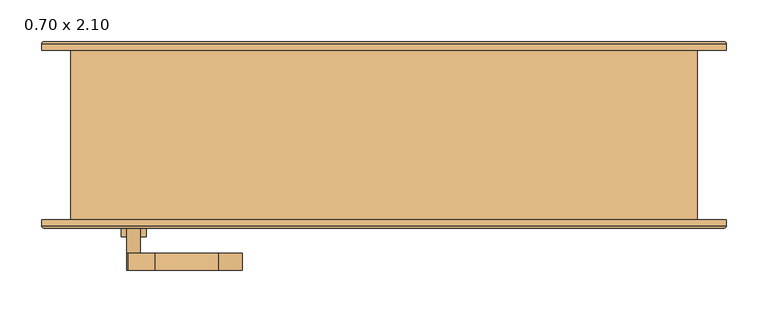
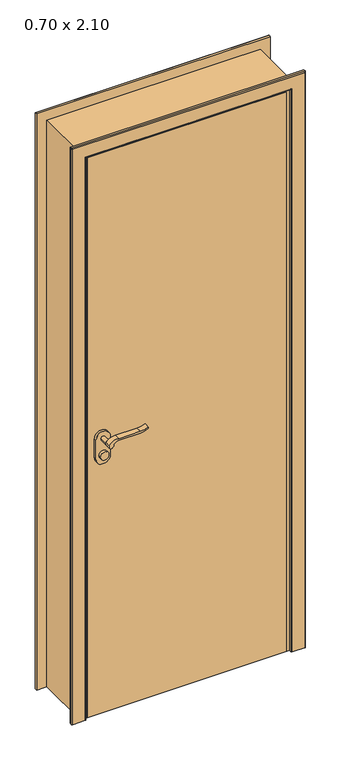
"""IFC4 building model written with IfcOpenShell, lengths in millimetres: door geometry, .CC_ND 300_PORTA SIMPLES DE ABRIR_COM EXTENSÃO : 0.70 x 2.10."""

from ifc_helpers import new_model, si_unit, point, frame, frame_2d, origin, origin_with_axes, place, context, project, spatial, polyline, circle_curve, ellipse_curve, trimmed, segment, composite_curve, outline, extrude, faceted_brep, source, transform, mapped, element, save
from ifc_brep_helpers import plane_surface, cylinder_surface, advanced_brep


def door_0_70_x_2_10_da532085(model_context):
    return source(origin(), model_context, "Body", "SolidModel", [
        extrude(outline(composite_curve([segment(trimmed(circle_curve(frame_2d((964.5, -300.0)), 15.0), [point((964.5, -285.0))], [point((964.5, -315.0))], False, "CARTESIAN"), True, "CONTINUOUS"), segment(trimmed(circle_curve(frame_2d((964.5, -300.0)), 15.0), [point((964.5, -315.0))], [point((964.5, -285.0))], False, "CARTESIAN"), True, "CONTINUOUS")], self_intersect=False)), frame((0.0, -136.4, 0.0), z_axis=(0.0, 1.0, 0.0), x_axis=(0.0, 0.0, 1.0)), (0.0, 0.0, 1.0), 10.0),
        extrude(outline(composite_curve([segment(trimmed(circle_curve(frame_2d((964.5, -300.0)), 15.0), [point((964.5, -285.0))], [point((964.5, -315.0))], False, "CARTESIAN"), True, "CONTINUOUS"), segment(trimmed(circle_curve(frame_2d((964.5, -300.0)), 15.0), [point((964.5, -315.0))], [point((964.5, -285.0))], False, "CARTESIAN"), True, "CONTINUOUS")], self_intersect=False)), frame((0.0, -76.4, 0.0), z_axis=(0.0, 1.0, 0.0), x_axis=(0.0, 0.0, 1.0)), (0.0, 0.0, 1.0), 10.0),
        extrude(outline(composite_curve([segment(trimmed(circle_curve(frame_2d((1024.5, -300.0)), 8.0), [point((1029.1523287, -306.5081363))], [point((1024.5, -292.0))], False, "CARTESIAN"), True, "CONTINUOUS"), segment(trimmed(circle_curve(frame_2d((1019.3738613, -274.6138099)), 18.1261387), [point((1024.5, -292.0))], [point((1037.5, -274.6138099))], True, "CARTESIAN"), True, "CONTINUOUS"), segment(polyline([(1037.5, -274.6138099), (1037.5, -198.3564091)]), True, "CONTINUOUS"), segment(trimmed(circle_curve(frame_2d((1096.7709207, -201.9396612)), 59.3791355), [point((1037.5, -198.3564091))], [point((1046.7135558, -170.0))], False, "CARTESIAN"), True, "CONTINUOUS"), segment(polyline([(1046.7135558, -170.0), (1049.5, -170.0)]), True, "CONTINUOUS"), segment(trimmed(circle_curve(frame_2d((1127.7850638, -198.4227909)), 83.2850902), [point((1049.5, -170.0))], [point((1044.5, -198.3564091))], True, "CARTESIAN"), True, "CONTINUOUS"), segment(polyline([(1044.5, -198.3564091), (1044.5, -274.6325667)]), True, "CONTINUOUS"), segment(trimmed(circle_curve(frame_2d((1007.2555521, -276.3324871)), 37.2832219), [point((1044.5, -274.6325667))], [point((1029.1523287, -306.5081363))], False, "CARTESIAN"), True, "CONTINUOUS")], self_intersect=False)), frame((0.0, -176.4, 0.0), z_axis=(0.0, 1.0, 0.0), x_axis=(0.0, 0.0, 1.0)), (0.0, 0.0, 1.0), 20.0),
        extrude(outline(composite_curve([segment(trimmed(circle_curve(frame_2d((1019.3738682, -274.6138122)), 18.1261318), [point((1024.4999903, -292.0))], [point((1037.5, -274.6138122))], True, "CARTESIAN"), True, "CONTINUOUS"), segment(polyline([(1037.5, -274.6138122), (1037.5, -198.3564091)]), True, "CONTINUOUS"), segment(trimmed(circle_curve(frame_2d((1096.7709207, -201.9396612)), 59.3791355), [point((1037.5, -198.3564091))], [point((1046.7135558, -170.0))], False, "CARTESIAN"), True, "CONTINUOUS"), segment(polyline([(1046.7135558, -170.0), (1049.5, -170.0)]), True, "CONTINUOUS"), segment(trimmed(circle_curve(frame_2d((1127.7850638, -198.4227909)), 83.2850902), [point((1049.5, -170.0))], [point((1044.5, -198.3564091))], True, "CARTESIAN"), True, "CONTINUOUS"), segment(polyline([(1044.5, -198.3564091), (1044.5, -274.6325667)]), True, "CONTINUOUS"), segment(trimmed(circle_curve(frame_2d((1007.2555521, -276.3324871)), 37.2832219), [point((1044.5, -274.6325667))], [point((1029.1523287, -306.5081363))], False, "CARTESIAN"), True, "CONTINUOUS"), segment(trimmed(circle_curve(frame_2d((1024.5, -300.0)), 8.0), [point((1029.1523287, -306.5081363))], [point((1024.4999903, -292.0))], False, "CARTESIAN"), True, "CONTINUOUS")], self_intersect=False)), frame((0.0, -46.4, 0.0), z_axis=(0.0, 1.0, 0.0), x_axis=(0.0, 0.0, 1.0)), (0.0, 0.0, 1.0), 20.0),
        extrude(outline(composite_curve([segment(trimmed(circle_curve(frame_2d((1024.5, -300.0)), 8.0), [point((1024.5, -292.0))], [point((1024.5, -308.0))], False, "CARTESIAN"), True, "CONTINUOUS"), segment(trimmed(circle_curve(frame_2d((1024.5, -300.0)), 8.0), [point((1024.5, -308.0))], [point((1024.5, -292.0))], False, "CARTESIAN"), True, "CONTINUOUS")], self_intersect=False)), frame((0.0, -156.4, 0.0), z_axis=(0.0, 1.0, 0.0), x_axis=(0.0, 0.0, 1.0)), (0.0, 0.0, 1.0), 30.0),
        extrude(outline(composite_curve([segment(trimmed(circle_curve(frame_2d((1024.5, -300.0)), 8.0), [point((1024.5, -292.0))], [point((1024.5, -308.0))], False, "CARTESIAN"), True, "CONTINUOUS"), segment(trimmed(circle_curve(frame_2d((1024.5, -300.0)), 8.0), [point((1024.5, -308.0))], [point((1024.5, -292.0))], False, "CARTESIAN"), True, "CONTINUOUS")], self_intersect=False)), frame((0.0, -76.4, 0.0), z_axis=(0.0, 1.0, 0.0), x_axis=(0.0, 0.0, 1.0)), (0.0, 0.0, 1.0), 30.0),
        extrude(outline(composite_curve([segment(trimmed(circle_curve(frame_2d((954.5, -300.0)), 25.0), [point((954.5, -325.0))], [point((954.5, -275.0))], False, "CARTESIAN"), True, "CONTINUOUS"), segment(polyline([(954.5, -275.0), (1024.5, -275.0)]), True, "CONTINUOUS"), segment(trimmed(circle_curve(frame_2d((1024.5, -300.0)), 25.0), [point((1024.5, -275.0))], [point((1024.5, -325.0))], False, "CARTESIAN"), True, "CONTINUOUS"), segment(polyline([(1024.5, -325.0), (954.5, -325.0)]), True, "CONTINUOUS")], self_intersect=False)), frame((0.0, -126.4, 0.0), z_axis=(0.0, 1.0, 0.0), x_axis=(0.0, 0.0, 1.0)), (0.0, 0.0, 1.0), 10.0),
        extrude(outline(composite_curve([segment(trimmed(circle_curve(frame_2d((954.5, -300.0)), 25.0), [point((954.5, -325.0))], [point((954.5, -275.0))], False, "CARTESIAN"), True, "CONTINUOUS"), segment(polyline([(954.5, -275.0), (1024.5, -275.0)]), True, "CONTINUOUS"), segment(trimmed(circle_curve(frame_2d((1024.5, -300.0)), 25.0), [point((1024.5, -275.0))], [point((1024.5, -325.0))], False, "CARTESIAN"), True, "CONTINUOUS"), segment(polyline([(1024.5, -325.0), (954.5, -325.0)]), True, "CONTINUOUS")], self_intersect=False)), frame((0.0, -86.4, 0.0), z_axis=(0.0, 1.0, 0.0), x_axis=(0.0, 0.0, 1.0)), (0.0, 0.0, 1.0), 10.0),
        faceted_brep([(342.0, 86.9, 0.0), (375.0, 86.9, 0.0), (375.0, -116.4, 0.0), (350.0, -116.4, 0.0), (350.0, -86.4, 0.0), (342.0, -86.4, 0.0), (342.0, 86.9, 2067.0), (-342.0, 86.9, 2067.0), (-342.0, 86.9, 0.0), (-375.0, 86.9, 0.0), (-375.0, 86.9, 2100.0), (375.0, 86.9, 2100.0), (375.0, -116.4, 2100.0), (-375.0, -116.4, 2100.0), (-375.0, -116.4, 0.0), (-350.0, -116.4, 0.0), (-350.0, -116.4, 2075.0), (350.0, -116.4, 2075.0), (350.0, -86.4, 2075.0), (-350.0, -86.4, 2075.0), (-350.0, -86.4, 0.0), (-342.0, -86.4, 0.0), (-342.0, -86.4, 2067.0), (342.0, -86.4, 2067.0)], [[[0, 1, 2, 3, 4, 5]], [[1, 0, 6, 7, 8, 9, 10, 11]], [[2, 1, 11, 12]], [[3, 2, 12, 13, 14, 15, 16, 17]], [[4, 3, 17, 18]], [[5, 4, 18, 19, 20, 21, 22, 23]], [[0, 5, 23, 6]], [[7, 22, 21, 8]], [[8, 21, 20, 15, 14, 9]], [[13, 10, 9, 14]], [[19, 16, 15, 20]], [[12, 11, 10, 13]], [[18, 17, 16, 19]], [[6, 23, 22, 7]]]),
        extrude(outline(polyline([(-350.0, -86.4), (350.0, -86.4), (350.0, -116.4), (-350.0, -116.4), (-350.0, -86.4)])), origin_with_axes(), (0.0, 0.0, 1.0), 2075.0),
        advanced_brep(
        [(-410.0, -116.4, 0.0), (-360.0, -116.4, 0.0), (-360.0, -123.4, 0.0), (-363.0, -126.4, 0.0), (-407.0, -126.4, 0.0), (-410.0, -123.4, 0.0), (-410.0, -116.4, 2135.0), (410.0, -116.4, 2135.0), (410.0, -116.4, 0.0), (360.0, -116.4, 0.0), (360.0, -116.4, 2085.0), (-360.0, -116.4, 2085.0), (-360.0, -123.4, 2085.0), (-363.0, -126.4, 2088.0), (363.0, -126.4, 2088.0), (363.0, -126.4, 0.0), (407.0, -126.4, 0.0), (407.0, -126.4, 2132.0), (-407.0, -126.4, 2132.0), (-410.0, -123.4, 2135.0), (410.0, -123.4, 2135.0), (410.0, -123.4, 0.0), (360.0, -123.4, 0.0), (360.0, -123.4, 2085.0)],
        [
            (0, 1),
            (1, 2),
            (2, 3, circle_curve(frame((-363.0, -123.4, 0.0), z_axis=(0.0, 0.0, -1.0), x_axis=(1.0, 0.0, 0.0)), 3.0)),
            (3, 4),
            (4, 5, circle_curve(frame((-407.0, -123.4, 0.0), z_axis=(0.0, 0.0, -1.0), x_axis=(1.0, 0.0, 0.0)), 3.0)),
            (5, 0),
            (0, 6),
            (6, 7),
            (7, 8),
            (8, 9),
            (9, 10),
            (10, 11),
            (11, 1),
            (11, 12),
            (12, 2),
            (12, 13, ellipse_curve(frame((-363.0, -123.4, 2088.0), z_axis=(-0.7071067811865475, 0.0, -0.7071067811865475), x_axis=(0.7071067811865474, 0.0, -0.7071067811865476)), 4.2426407, 3.0)),
            (13, 3),
            (13, 14),
            (14, 15),
            (15, 16),
            (16, 17),
            (17, 18),
            (18, 4),
            (18, 19, ellipse_curve(frame((-407.0, -123.4, 2132.0), z_axis=(-0.7071067811865475, 0.0, -0.7071067811865475), x_axis=(0.7071067811865474, 0.0, -0.7071067811865476)), 4.2426407, 3.0)),
            (19, 5),
            (19, 6),
            (7, 20),
            (20, 21),
            (21, 8),
            (21, 16, circle_curve(frame((407.0, -123.4, 0.0), z_axis=(0.0, 0.0, -1.0), x_axis=(-1.0, 0.0, 0.0)), 3.0)),
            (15, 22, circle_curve(frame((363.0, -123.4, 0.0), z_axis=(0.0, 0.0, -1.0), x_axis=(-1.0, 0.0, 0.0)), 3.0)),
            (22, 9),
            (23, 10),
            (22, 23),
            (14, 23, ellipse_curve(frame((363.0, -123.4, 2088.0), z_axis=(0.7071067811865475, 0.0, -0.7071067811865475), x_axis=(0.7071067811865474, 0.0, 0.7071067811865476)), 4.2426407, 3.0)),
            (20, 17, ellipse_curve(frame((407.0, -123.4, 2132.0), z_axis=(0.7071067811865475, 0.0, -0.7071067811865475), x_axis=(0.7071067811865474, 0.0, 0.7071067811865476)), 4.2426407, 3.0)),
            (23, 12),
            (19, 20),
        ],
        [
            plane_surface(frame((-360.0, -116.4, 0.0), z_axis=(0.0, 0.0, -1.0), x_axis=(0.0, 1.0, 0.0))),
            plane_surface(frame((-410.0, -116.4, 0.0), z_axis=(0.0, 1.0, 0.0), x_axis=(0.0, 0.0, 1.0))),
            plane_surface(frame((-360.0, -116.4, 0.0), z_axis=(1.0, 0.0, 0.0), x_axis=(0.0, 0.0, 1.0))),
            cylinder_surface(frame((-363.0, -123.4, 0.0), z_axis=(0.0, 0.0, -1.0), x_axis=(1.0, 0.0, 0.0)), 3.0),
            plane_surface(frame((-363.0, -126.4, 0.0), z_axis=(0.0, -1.0, 0.0), x_axis=(0.0, 0.0, 1.0))),
            cylinder_surface(frame((-407.0, -123.4, 0.0), z_axis=(0.0, 0.0, -1.0), x_axis=(1.0, 0.0, 0.0)), 3.0),
            plane_surface(frame((-410.0, -123.4, 0.0), z_axis=(-1.0, 0.0, 0.0), x_axis=(0.0, 0.0, 1.0))),
            plane_surface(frame((410.0, -123.4, 2135.0), z_axis=(1.0, 0.0, 0.0), x_axis=(0.0, 0.0, -1.0))),
            plane_surface(frame((360.0, -116.4, 0.0), z_axis=(0.0, 0.0, -1.0), x_axis=(0.0, 1.0, 0.0))),
            plane_surface(frame((360.0, -116.4, 2085.0), z_axis=(-1.0, 0.0, 0.0), x_axis=(0.0, 0.0, -1.0))),
            cylinder_surface(frame((363.0, -123.4, 2085.0), z_axis=(0.0, 0.0, 1.0), x_axis=(-1.0, 0.0, 0.0)), 3.0),
            cylinder_surface(frame((407.0, -123.4, 2085.0), z_axis=(0.0, 0.0, 1.0), x_axis=(-1.0, 0.0, 0.0)), 3.0),
            plane_surface(frame((-360.0, -116.4, 2085.0), z_axis=(0.0, 0.0, -1.0), x_axis=(1.0, 0.0, 0.0))),
            plane_surface(frame((-410.0, -123.4, 2135.0), z_axis=(0.0, 0.0, 1.0), x_axis=(1.0, 0.0, 0.0))),
            cylinder_surface(frame((-360.0, -123.4, 2088.0), z_axis=(-1.0, 0.0, 0.0), x_axis=(0.0, 0.0, -1.0)), 3.0),
            cylinder_surface(frame((-360.0, -123.4, 2132.0), z_axis=(-1.0, 0.0, 0.0), x_axis=(0.0, 0.0, -1.0)), 3.0),
        ],
        [
            (0, [[1, 2, 3, 4, 5, 6]]),
            (1, [[-1, 7, 8, 9, 10, 11, 12, 13]]),
            (2, [[-2, -13, 14, 15]]),
            (3, [[-3, -15, 16, 17]]),
            (4, [[-4, -17, 18, 19, 20, 21, 22, 23]]),
            (5, [[-5, -23, 24, 25]]),
            (6, [[-6, -25, 26, -7]]),
            (7, [[27, 28, 29, -9]]),
            (8, [[-29, 30, -20, 31, 32, -10]]),
            (9, [[33, -11, -32, 34]]),
            (10, [[35, -34, -31, -19]]),
            (11, [[36, -21, -30, -28]]),
            (12, [[-14, -12, -33, 37]]),
            (13, [[-26, 38, -27, -8]]),
            (14, [[-16, -37, -35, -18]]),
            (15, [[-24, -22, -36, -38]]),
        ],
    ),
        advanced_brep(
        [(410.0, 86.9, 0.0), (360.0, 86.9, 0.0), (360.0, 93.9157283, 0.0), (362.9842717, 96.9, 0.0), (407.0342217, 96.9, 0.0), (410.0, 93.9342217, 0.0), (410.0, 86.9, 2135.0), (-410.0, 86.9, 2135.0), (-410.0, 86.9, 0.0), (-360.0, 86.9, 0.0), (-360.0, 86.9, 2085.0), (360.0, 86.9, 2085.0), (360.0, 93.9157283, 2085.0), (362.9842717, 96.9, 2087.9842717), (-362.9842717, 96.9, 2087.9842717), (-362.9842717, 96.9, 0.0), (-407.0342217, 96.9, 0.0), (-407.0342217, 96.9, 2132.0342217), (407.0342217, 96.9, 2132.0342217), (410.0, 93.9342217, 2135.0), (-410.0, 93.9342217, 2135.0), (-410.0, 93.9342217, 0.0), (-360.0, 93.9157283, 0.0), (-360.0, 93.9157283, 2085.0)],
        [
            (0, 1),
            (1, 2),
            (2, 3, circle_curve(frame((362.9842717, 93.9157283, 0.0), z_axis=(0.0, 0.0, -1.0), x_axis=(1.0, 0.0, 0.0)), 2.9842717)),
            (3, 4),
            (4, 5, circle_curve(frame((407.0342217, 93.9342217, 0.0), z_axis=(0.0, 0.0, -1.0), x_axis=(1.0, 0.0, 0.0)), 2.9657783)),
            (5, 0),
            (0, 6),
            (6, 7),
            (7, 8),
            (8, 9),
            (9, 10),
            (10, 11),
            (11, 1),
            (11, 12),
            (12, 2),
            (12, 13, ellipse_curve(frame((362.9842717, 93.9157283, 2087.9842717), z_axis=(0.7071067811865475, 0.0, -0.7071067811865475), x_axis=(-0.7071067811865474, 0.0, -0.7071067811865476)), 4.2203975, 2.9842717)),
            (13, 3),
            (13, 14),
            (14, 15),
            (15, 16),
            (16, 17),
            (17, 18),
            (18, 4),
            (18, 19, ellipse_curve(frame((407.0342217, 93.9342217, 2132.0342217), z_axis=(0.7071067811865475, 0.0, -0.7071067811865475), x_axis=(-0.7071067811865474, 0.0, -0.7071067811865476)), 4.1942438, 2.9657783)),
            (19, 5),
            (19, 6),
            (7, 20),
            (20, 21),
            (21, 8),
            (21, 16, circle_curve(frame((-407.0342217, 93.9342217, 0.0), z_axis=(0.0, 0.0, -1.0), x_axis=(-1.0, 0.0, 0.0)), 2.9657783)),
            (15, 22, circle_curve(frame((-362.9842717, 93.9157283, 0.0), z_axis=(0.0, 0.0, -1.0), x_axis=(-1.0, 0.0, 0.0)), 2.9842717)),
            (22, 9),
            (23, 10),
            (22, 23),
            (14, 23, ellipse_curve(frame((-362.9842717, 93.9157283, 2087.9842717), z_axis=(-0.7071067811865475, 0.0, -0.7071067811865475), x_axis=(-0.7071067811865474, 0.0, 0.7071067811865476)), 4.2203975, 2.9842717)),
            (20, 17, ellipse_curve(frame((-407.0342217, 93.9342217, 2132.0342217), z_axis=(-0.7071067811865475, 0.0, -0.7071067811865475), x_axis=(-0.7071067811865474, 0.0, 0.7071067811865476)), 4.1942438, 2.9657783)),
            (23, 12),
            (19, 20),
        ],
        [
            plane_surface(frame((360.0, 86.9, 0.0), z_axis=(0.0, 0.0, -1.0), x_axis=(0.0, 1.0, 0.0))),
            plane_surface(frame((410.0, 86.9, 0.0), z_axis=(0.0, -1.0, 0.0), x_axis=(0.0, 0.0, 1.0))),
            plane_surface(frame((360.0, 86.9, 0.0), z_axis=(-1.0, 0.0, 0.0), x_axis=(0.0, 0.0, 1.0))),
            cylinder_surface(frame((362.9842717, 93.9157283, 0.0), z_axis=(0.0, 0.0, -1.0), x_axis=(1.0, 0.0, 0.0)), 2.9842717),
            plane_surface(frame((362.9842717, 96.9, 0.0), z_axis=(0.0, 1.0, 0.0), x_axis=(0.0, 0.0, 1.0))),
            cylinder_surface(frame((407.0342217, 93.9342217, 0.0), z_axis=(0.0, 0.0, -1.0), x_axis=(1.0, 0.0, 0.0)), 2.9657783),
            plane_surface(frame((410.0, 93.9342217, 0.0), z_axis=(1.0, 0.0, 0.0), x_axis=(0.0, 0.0, 1.0))),
            plane_surface(frame((-410.0, 93.9342217, 2135.0), z_axis=(-1.0, 0.0, 0.0), x_axis=(0.0, 0.0, -1.0))),
            plane_surface(frame((-360.0, 86.9, 0.0), z_axis=(0.0, 0.0, -1.0), x_axis=(0.0, 1.0, 0.0))),
            plane_surface(frame((-360.0, 86.9, 2085.0), z_axis=(1.0, 0.0, 0.0), x_axis=(0.0, 0.0, -1.0))),
            cylinder_surface(frame((-362.9842717, 93.9157283, 2085.0), z_axis=(0.0, 0.0, 1.0), x_axis=(-1.0, 0.0, 0.0)), 2.9842717),
            cylinder_surface(frame((-407.0342217, 93.9342217, 2085.0), z_axis=(0.0, 0.0, 1.0), x_axis=(-1.0, 0.0, 0.0)), 2.9657783),
            plane_surface(frame((360.0, 86.9, 2085.0), z_axis=(0.0, 0.0, -1.0), x_axis=(-1.0, 0.0, 0.0))),
            plane_surface(frame((410.0, 93.9342217, 2135.0), z_axis=(0.0, 0.0, 1.0), x_axis=(-1.0, 0.0, 0.0))),
            cylinder_surface(frame((360.0, 93.9157283, 2087.9842717), z_axis=(1.0, 0.0, 0.0), x_axis=(0.0, 0.0, 1.0)), 2.9842717),
            cylinder_surface(frame((360.0, 93.9342217, 2132.0342217), z_axis=(1.0, 0.0, 0.0), x_axis=(0.0, 0.0, 1.0)), 2.9657783),
        ],
        [
            (0, [[1, 2, 3, 4, 5, 6]]),
            (1, [[-1, 7, 8, 9, 10, 11, 12, 13]]),
            (2, [[-2, -13, 14, 15]]),
            (3, [[-3, -15, 16, 17]]),
            (4, [[-4, -17, 18, 19, 20, 21, 22, 23]]),
            (5, [[-5, -23, 24, 25]]),
            (6, [[-6, -25, 26, -7]]),
            (7, [[27, 28, 29, -9]]),
            (8, [[-29, 30, -20, 31, 32, -10]]),
            (9, [[33, -11, -32, 34]]),
            (10, [[35, -34, -31, -19]]),
            (11, [[36, -21, -30, -28]]),
            (12, [[-14, -12, -33, 37]]),
            (13, [[-26, 38, -27, -8]]),
            (14, [[-16, -37, -35, -18]]),
            (15, [[-24, -22, -36, -38]]),
        ],
    ),
    ])


if __name__ == "__main__":
    model = new_model("IFC4")
    model_context = context("Model", 3, world=origin())
    ifc_project = project(units=[si_unit("LENGTHUNIT", "METRE", prefix="MILLI")], contexts=[model_context])
    site = spatial("IfcSite", under=ifc_project)
    building = spatial("IfcBuilding", under=site)
    placement = place(None, origin())
    door_0_70_x_2_10_shape = door_0_70_x_2_10_da532085(model_context)
    element("IfcDoor", 1, ObjectType=".CC_ND 300_PORTA SIMPLES DE ABRIR_COM EXTENSÃO : 0.70 x 2.10", at=placement, inside=building, context=model_context, shape_type="MappedRepresentation", body=[
        mapped(door_0_70_x_2_10_shape, transform((0.0, 0.0, 0.0), x_axis=(1.0, 0.0, 0.0), y_axis=(0.0, 1.0, 0.0), z_axis=(0.0, 0.0, 1.0))),
    ])
    save(model, "model.ifc")

# Revit data of these elements
# Type ".CC_ND 300_PORTA SIMPLES DE ABRIR_COM EXTENSÃO : 0.70 x 2.10"
#   Type Mark = "155"
#   Analytic Construction = "<None>"
#   Rough Width = 0.75 m
#   Espessura moldura externa = 0.01 m
#   Espessura moldura interna = 0.01 m
#   Largura moldura = 0.05 m
#   Extensão acabamento exterior [instance default] = 0.00 m
#   Extensão acabamento interior [instance default] = 0.00 m
#   Espessura batente = 0.025 m
#   Thickness = 0.03 m
#   Altura batente = 2.085 m
#   Aux Arco [instance default] = 0.70 m
#   Rough Height = 2.125 m
#   Height = 2.10 m
#   Width = 0.70 m
#   Moldura interna [instance default] = yes
#   Moldura externa [instance default] = yes
#   Porta = .MADEIRA COM PINTURA ESMALTE BRANCO ACETINADO
#   Moldura = .MADEIRA COM PINTURA ESMALTE BRANCO ACETINADO
#   Maçaneta = .ALUMÍNIO
#   Batente = .MADEIRA COM PINTURA ESMALTE BRANCO ACETINADO
#   Function = (empty or 0)
#   Wall Closure = (empty or 0)
# Element 1 (IfcDoor, ".CC_ND 300_PORTA SIMPLES DE ABRIR_COM EXTENSÃO : 0.70 x 2.10")
#   Extensão acabamento interior = 0.0295 m
#   Aux Arco = 0.7295 m
#   Materials on its faces: ".MADEIRA COM PINTURA ESMALTE BRANCO ACETINADO", ".ALUMÍNIO"
# Materials
#   ".MADEIRA COM PINTURA ESMALTE BRANCO ACETINADO": class ".CC_MADEIRAS", colour RGB 240 240 240, transparency 0, Description = "Madeira com pintura esmalte branco acetinado.", Cost = 0
#   ".ALUMÍNIO": class "CC_METAIS", colour RGB 244 244 244, transparency 0, Description = "Material alumínio", Cost = 0
